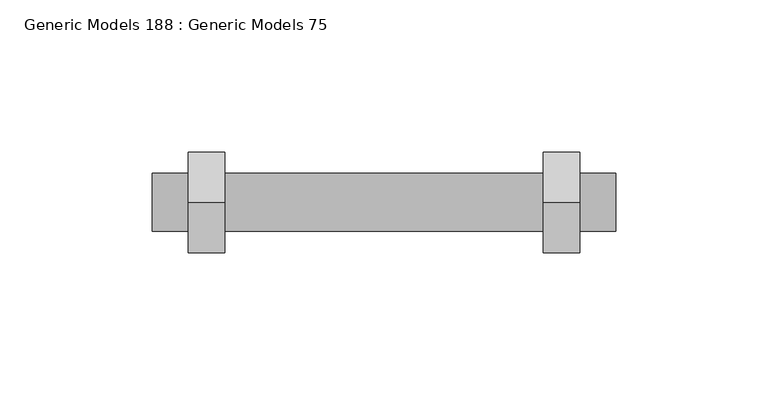
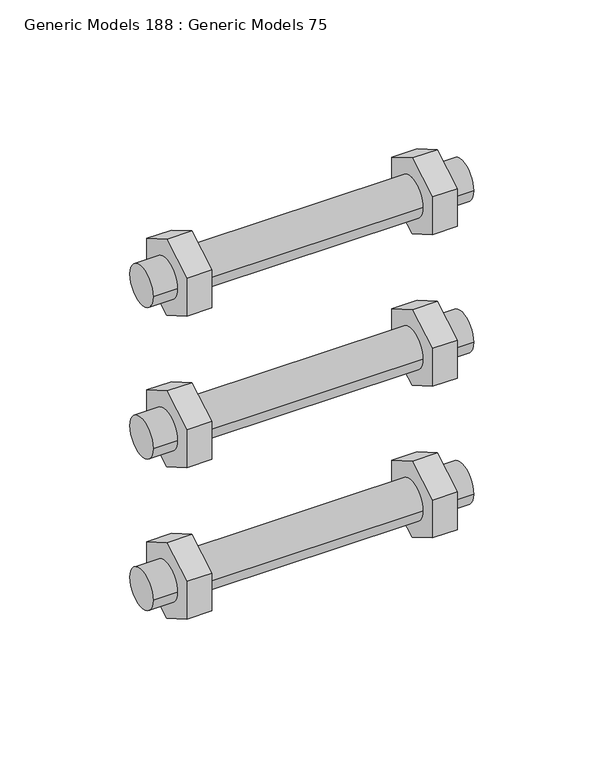
"""IFC4 building model written with IfcOpenShell, lengths in millimetres: proxy geometry, Generic Models 188 : Generic Models 75."""

from ifc_helpers import new_model, si_unit, point, frame, frame_2d, origin, place, context, project, spatial, polyline, circle_curve, trimmed, segment, composite_curve, outline, extrude, source, transform, mapped, element, save


def generic_models_188_generic_models_75_ffbcfaf3(model_context):
    return source(origin(), model_context, "Body", "SweptSolid", [
        extrude(outline(polyline([(36269.1373281, 269062.859622), (36269.1373281, 269043.809622), (36252.6395442, 269034.284622), (36236.1417603, 269043.809622), (36236.1417603, 269062.859622), (36252.6395442, 269072.384622), (36269.1373281, 269062.859622)])), frame((31918.2596032, 0.0, 0.0), z_axis=(1.0, 0.0, 0.0), x_axis=(0.0, 1.0, 0.0)), (0.0, 0.0, 1.0), 11.90625),
        extrude(outline(polyline([(36269.1373281, 268986.659622), (36269.1373281, 268967.609622), (36252.6395442, 268958.084622), (36236.1417603, 268967.609622), (36236.1417603, 268986.659622), (36252.6395442, 268996.184622), (36269.1373281, 268986.659622)])), frame((31918.2596032, 0.0, 0.0), z_axis=(1.0, 0.0, 0.0), x_axis=(0.0, 1.0, 0.0)), (0.0, 0.0, 1.0), 11.90625),
        extrude(outline(polyline([(36269.1373281, 268910.459622), (36269.1373281, 268891.409622), (36252.6395442, 268881.884622), (36236.1417603, 268891.409622), (36236.1417603, 268910.459622), (36252.6395442, 268919.984622), (36269.1373281, 268910.459622)])), frame((31918.2596032, 0.0, 0.0), z_axis=(1.0, 0.0, 0.0), x_axis=(0.0, 1.0, 0.0)), (0.0, 0.0, 1.0), 11.90625),
        extrude(outline(polyline([(36269.1373281, 269062.859622), (36269.1373281, 269043.809622), (36252.6395442, 269034.284622), (36236.1417603, 269043.809622), (36236.1417603, 269062.859622), (36252.6395442, 269072.384622), (36269.1373281, 269062.859622)])), frame((31801.5783532, 0.0, 0.0), z_axis=(1.0, 0.0, 0.0), x_axis=(0.0, 1.0, 0.0)), (0.0, 0.0, 1.0), 11.90625),
        extrude(outline(polyline([(36269.1373281, 268986.659622), (36269.1373281, 268967.609622), (36252.6395442, 268958.084622), (36236.1417603, 268967.609622), (36236.1417603, 268986.659622), (36252.6395442, 268996.184622), (36269.1373281, 268986.659622)])), frame((31801.5783532, 0.0, 0.0), z_axis=(1.0, 0.0, 0.0), x_axis=(0.0, 1.0, 0.0)), (0.0, 0.0, 1.0), 11.90625),
        extrude(outline(polyline([(36269.1373281, 268910.459622), (36269.1373281, 268891.409622), (36252.6395442, 268881.884622), (36236.1417603, 268891.409622), (36236.1417603, 268910.459622), (36252.6395442, 268919.984622), (36269.1373281, 268910.459622)])), frame((31801.5783532, 0.0, 0.0), z_axis=(1.0, 0.0, 0.0), x_axis=(0.0, 1.0, 0.0)), (0.0, 0.0, 1.0), 11.90625),
        extrude(outline(composite_curve([segment(trimmed(circle_curve(frame_2d((36252.6395442, 268977.134622)), 9.525), [point((36243.1145442, 268977.134622))], [point((36262.1645442, 268977.134622))], False, "CARTESIAN"), True, "CONTINUOUS"), segment(trimmed(circle_curve(frame_2d((36252.6395442, 268977.134622)), 9.525), [point((36262.1645442, 268977.134622))], [point((36243.1145442, 268977.134622))], False, "CARTESIAN"), True, "CONTINUOUS")], self_intersect=False)), frame((31789.6721032, 0.0, 0.0), z_axis=(1.0, 0.0, 0.0), x_axis=(0.0, 1.0, 0.0)), (0.0, 0.0, 1.0), 152.4),
        extrude(outline(composite_curve([segment(trimmed(circle_curve(frame_2d((36252.6395442, 268900.934622)), 9.525), [point((36243.1145442, 268900.934622))], [point((36262.1645442, 268900.934622))], False, "CARTESIAN"), True, "CONTINUOUS"), segment(trimmed(circle_curve(frame_2d((36252.6395442, 268900.934622)), 9.525), [point((36262.1645442, 268900.934622))], [point((36243.1145442, 268900.934622))], False, "CARTESIAN"), True, "CONTINUOUS")], self_intersect=False)), frame((31789.6721032, 0.0, 0.0), z_axis=(1.0, 0.0, 0.0), x_axis=(0.0, 1.0, 0.0)), (0.0, 0.0, 1.0), 152.4),
        extrude(outline(composite_curve([segment(trimmed(circle_curve(frame_2d((36252.6395442, 269053.334622)), 9.525), [point((36243.1145442, 269053.334622))], [point((36262.1645442, 269053.334622))], False, "CARTESIAN"), True, "CONTINUOUS"), segment(trimmed(circle_curve(frame_2d((36252.6395442, 269053.334622)), 9.525), [point((36262.1645442, 269053.334622))], [point((36243.1145442, 269053.334622))], False, "CARTESIAN"), True, "CONTINUOUS")], self_intersect=False)), frame((31789.6721032, 0.0, 0.0), z_axis=(1.0, 0.0, 0.0), x_axis=(0.0, 1.0, 0.0)), (0.0, 0.0, 1.0), 152.4),
    ])


if __name__ == "__main__":
    model = new_model("IFC4")
    model_context = context("Model", 3, world=origin())
    ifc_project = project(units=[si_unit("LENGTHUNIT", "METRE", prefix="MILLI")], contexts=[model_context])
    site = spatial("IfcSite", under=ifc_project)
    building = spatial("IfcBuilding", under=site)
    placement = place(None, origin())
    generic_models_188_generic_models_75_shape = generic_models_188_generic_models_75_ffbcfaf3(model_context)
    element("IfcBuildingElementProxy", 1, Name="Generic Models 188 : Generic Models 75", ObjectType="Generic Models 188 : Generic Models 75", at=placement, inside=building, context=model_context, shape_type="MappedRepresentation", body=[
        mapped(generic_models_188_generic_models_75_shape, transform((0.0, 0.0, 0.0), x_axis=(1.0, 0.0, 0.0), y_axis=(0.0, 1.0, 0.0), z_axis=(0.0, 0.0, 1.0))),
    ])
    save(model, "model.ifc")
